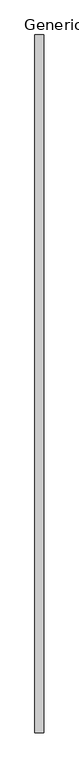
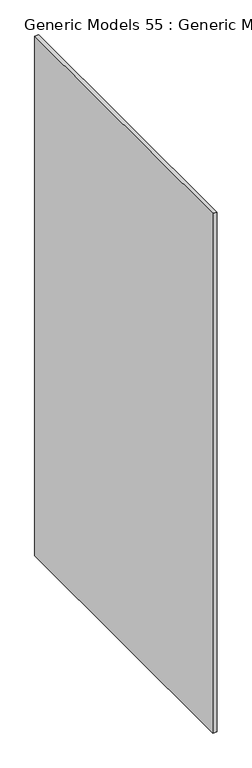
"""IFC4 building model written with IfcOpenShell, lengths in millimetres: proxy geometry, Generic Models 55 : Generic Models 1."""

import ifcopenshell
import ifcopenshell.guid

model = None  # the IFC model being written
_history = None  # IfcOwnerHistory: only IFC2X3 demands one
_inside = {}  # id of a spatial element -> (the spatial element, [elements in it])
_under = {}  # id of a project, library or spatial element -> (it, [spatial elements below it])
_declared = {}  # id of a project -> (the project, [libraries it declares])
_typed = {}  # id of a type object -> (the type object, [elements of that type])
_made_of = {}  # id of a material, layer set ... -> (it, [elements and type objects made of it])


def new_model(schema):
    """Start an empty IFC model of exactly this schema.

    Asked for "IFC4X3", IfcOpenShell would pick the latest addendum, in which some entities
    have other attributes; the version numbers below select the first issue.
    IFC2X3 requires an IfcOwnerHistory on every rooted entity: one is made here for all.
    """
    global model, _history
    if schema == "IFC4X3":
        model = ifcopenshell.file(schema_version=(4, 3, 0, 0))
    else:
        model = ifcopenshell.file(schema=schema)
    _inside.clear()
    _under.clear()
    _declared.clear()
    _typed.clear()
    _made_of.clear()
    _history = None
    if model.schema == "IFC2X3":
        org = make("IfcOrganization", Name="unknown")
        user = make(
            "IfcPersonAndOrganization",
            ThePerson=make("IfcPerson", FamilyName="unknown"),
            TheOrganization=org,
        )
        app = make(
            "IfcApplication",
            ApplicationDeveloper=org,
            Version="unknown",
            ApplicationFullName="unknown",
            ApplicationIdentifier="unknown",
        )
        _history = make(
            "IfcOwnerHistory",
            OwningUser=user,
            OwningApplication=app,
            ChangeAction="ADDED",
            CreationDate=0,
        )
    return model


def make(cls, **values):
    """One entity of the class cls with the attributes given. An attribute that is None is left unset."""
    return model.create_entity(
        cls, **{name: value for name, value in values.items() if value is not None}
    )


def rooted(cls, **values):
    """An entity with a GlobalId (a new one), such as an element, a storey or a relation."""
    return make(cls, GlobalId=ifcopenshell.guid.new(), OwnerHistory=_history, **values)


def si_unit(unit_type, name, prefix=None):
    """IfcSIUnit, for example si_unit("LENGTHUNIT", "METRE", prefix="MILLI")."""
    return make("IfcSIUnit", UnitType=unit_type, Prefix=prefix, Name=name)


def assignment(units):
    """IfcUnitAssignment: the units of a project."""
    return None if units is None else make("IfcUnitAssignment", Units=units)


def point(xyz):
    """IfcCartesianPoint."""
    return None if xyz is None else make("IfcCartesianPoint", Coordinates=xyz)


def direction(xyz):
    """IfcDirection."""
    return None if xyz is None else make("IfcDirection", DirectionRatios=xyz)


def frame(location, z_axis=None, x_axis=None):
    """IfcAxis2Placement3D, a coordinate frame: its origin and axes. An axis left out is left unset."""
    return make(
        "IfcAxis2Placement3D",
        Location=point(location),
        Axis=direction(z_axis),
        RefDirection=direction(x_axis),
    )


def origin():
    """The frame at (0, 0, 0) with its axes left unset."""
    return frame((0.0, 0.0, 0.0))


def place(relative_to, where):
    """IfcLocalPlacement: puts the frame where relative to a parent placement (None: the world)."""
    return make(
        "IfcLocalPlacement", PlacementRelTo=relative_to, RelativePlacement=where
    )


def context(
    kind, dimensions, precision=None, world=None, true_north=None, identifier=None
):
    """IfcGeometricRepresentationContext, for example the 3D "Model" context."""
    return make(
        "IfcGeometricRepresentationContext",
        ContextIdentifier=identifier,
        ContextType=kind,
        CoordinateSpaceDimension=dimensions,
        Precision=precision,
        WorldCoordinateSystem=world,
        TrueNorth=true_north,
    )


def project(units=None, contexts=None):
    """IfcProject with its units and contexts."""
    return rooted(
        "IfcProject",
        Name="project",
        RepresentationContexts=contexts,
        UnitsInContext=assignment(units),
    )


def spatial(cls, under=None, at=None, **own):
    """A site, building, storey or space (cls), placed at a placement, below another one or the project."""
    s = rooted(cls, ObjectPlacement=at, **own)
    if under is not None:
        _under.setdefault(under.id(), (under, []))[1].append(s)
    return s


def polyline(points):
    """IfcPolyline through the points."""
    return make("IfcPolyline", Points=[point(p) for p in points])


def outline(outer, holes=None, kind="AREA"):
    """IfcArbitraryClosedProfileDef: a profile drawn as a closed curve; with holes, ...WithVoids."""
    if holes is None:
        return make("IfcArbitraryClosedProfileDef", ProfileType=kind, OuterCurve=outer)
    return make(
        "IfcArbitraryProfileDefWithVoids",
        ProfileType=kind,
        OuterCurve=outer,
        InnerCurves=holes,
    )


def extrude(swept, where, along, depth):
    """IfcExtrudedAreaSolid: the profile swept, set in the frame where, extruded along a direction by depth."""
    return make(
        "IfcExtrudedAreaSolid",
        SweptArea=swept,
        Position=where,
        ExtrudedDirection=direction(along),
        Depth=depth,
    )


def shape(context_of_items, identifier, shape_type, items):
    """IfcShapeRepresentation: the items that make up one representation, for example the "Body"."""
    return make(
        "IfcShapeRepresentation",
        ContextOfItems=context_of_items,
        RepresentationIdentifier=identifier,
        RepresentationType=shape_type,
        Items=items,
    )


def source(mapping_origin, context_of_items, identifier, shape_type, items):
    """IfcRepresentationMap: a shape defined once, which mapped items show again and again."""
    return make(
        "IfcRepresentationMap",
        MappingOrigin=mapping_origin,
        MappedRepresentation=shape(context_of_items, identifier, shape_type, items),
    )


def transform(
    local_origin,
    x_axis=None,
    y_axis=None,
    z_axis=None,
    scale=None,
    scale2=None,
    scale3=None,
    uniform=True,
):
    """IfcCartesianTransformationOperator3D, or its non-uniform kind. x_axis, y_axis, z_axis: its Axis1, 2, 3."""
    if uniform:
        return make(
            "IfcCartesianTransformationOperator3D",
            Axis1=direction(x_axis),
            Axis2=direction(y_axis),
            LocalOrigin=point(local_origin),
            Scale=scale,
            Axis3=direction(z_axis),
        )
    return make(
        "IfcCartesianTransformationOperator3DnonUniform",
        Axis1=direction(x_axis),
        Axis2=direction(y_axis),
        LocalOrigin=point(local_origin),
        Scale=scale,
        Axis3=direction(z_axis),
        Scale2=scale2,
        Scale3=scale3,
    )


def mapped(mapping_source, mapping_target):
    """IfcMappedItem: shows the shape of a source again, moved by a transform."""
    return make(
        "IfcMappedItem", MappingSource=mapping_source, MappingTarget=mapping_target
    )


def made_of(thing, what):
    """Note that an element or type object is made of a material, layer set ...; save() writes the relation."""
    if what is not None:
        _made_of.setdefault(what.id(), (what, []))[1].append(thing)
    return thing


def element(
    cls,
    number,
    at=None,
    inside=None,
    cuts=None,
    type_object=None,
    material=None,
    context=None,
    identifier="Body",
    shape_type=None,
    held_by="IfcProductDefinitionShape",
    body=None,
    shapes=None,
    **own,
):
    """One element of the class cls, such as IfcWall. Its Tag is "e" and its number.

    at: its placement. inside: the storey or other place that contains it. cuts: it is an
    opening in that element (IfcRelVoidsElement). A single representation is given by context,
    identifier, shape_type and body (its items); several are given by shapes. held_by: the class
    of the entity that holds the representations. save() writes the other relations.
    """
    e = rooted(cls, Tag="e%d" % number, ObjectPlacement=at, **own)
    if body is not None:
        shapes = [shape(context, identifier, shape_type, body)]
    if shapes is not None:
        e.Representation = make(held_by, Representations=shapes)
    if inside is not None:
        _inside.setdefault(inside.id(), (inside, []))[1].append(e)
    if cuts is not None:
        rooted(
            "IfcRelVoidsElement", RelatingBuildingElement=cuts, RelatedOpeningElement=e
        )
    if type_object is not None:
        _typed.setdefault(type_object.id(), (type_object, []))[1].append(e)
    return made_of(e, material)


def aggregate(whole, parts):
    """IfcRelAggregates: a whole, such as a stair, and the parts it consists of."""
    return rooted("IfcRelAggregates", RelatingObject=whole, RelatedObjects=parts)


def save(model, path):
    """Write the relations noted so far, then the file.

    IfcRelAggregates (storeys below a building ...), IfcRelContainedInSpatialStructure (elements
    in a storey), IfcRelDefinesByType, IfcRelAssociatesMaterial and IfcRelDeclares: one each for
    every whole, place, type object, material and project.
    """
    for whole, parts in _under.values():
        aggregate(whole, parts)
    for where, things in _inside.values():
        rooted(
            "IfcRelContainedInSpatialStructure",
            RelatedElements=things,
            RelatingStructure=where,
        )
    for kind, things in _typed.values():
        rooted("IfcRelDefinesByType", RelatedObjects=things, RelatingType=kind)
    for what, things in _made_of.values():
        rooted("IfcRelAssociatesMaterial", RelatedObjects=things, RelatingMaterial=what)
    for by, libraries in _declared.values():
        rooted("IfcRelDeclares", RelatingContext=by, RelatedDefinitions=libraries)
    model.write(path)


def generic_models_55_generic_models_1_42571d6e(model_context):
    return source(origin(), model_context, "Body", "SweptSolid", [
        extrude(outline(polyline([(52238.275, 1219.2), (52238.275, 0.0), (52222.4, 0.0), (52222.4, 1219.2), (52238.275, 1219.2)])), frame((0.0, 0.0, 3054.35), z_axis=(0.0, 0.0, 1.0), x_axis=(1.0, 0.0, 0.0)), (0.0, 0.0, 1.0), 2168.128125),
    ])


if __name__ == "__main__":
    model = new_model("IFC4")
    model_context = context("Model", 3, world=origin())
    ifc_project = project(units=[si_unit("LENGTHUNIT", "METRE", prefix="MILLI")], contexts=[model_context])
    site = spatial("IfcSite", under=ifc_project)
    building = spatial("IfcBuilding", under=site)
    placement = place(None, origin())
    generic_models_55_generic_models_1_shape = generic_models_55_generic_models_1_42571d6e(model_context)
    element("IfcBuildingElementProxy", 1, Name="Generic Models 55 : Generic Models 1", ObjectType="Generic Models 55 : Generic Models 1", at=placement, inside=building, context=model_context, shape_type="MappedRepresentation", body=[
        mapped(generic_models_55_generic_models_1_shape, transform((0.0, 0.0, 0.0), x_axis=(1.0, 0.0, 0.0), y_axis=(0.0, 1.0, 0.0), z_axis=(0.0, 0.0, 1.0))),
    ])
    save(model, "model.ifc")

# Revit data of these elements
# Element 1 (IfcBuildingElementProxy, "Generic Models 55 : Generic Models 1")
#   Materials on its faces: "5/8\" GYP. BD"
# Materials
#   "5/8\" GYP. BD": class "Generic", colour RGB 255 255 255, transparency 0, Description = "Gypsum Wall Board", Cost = 0
